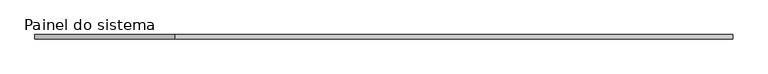
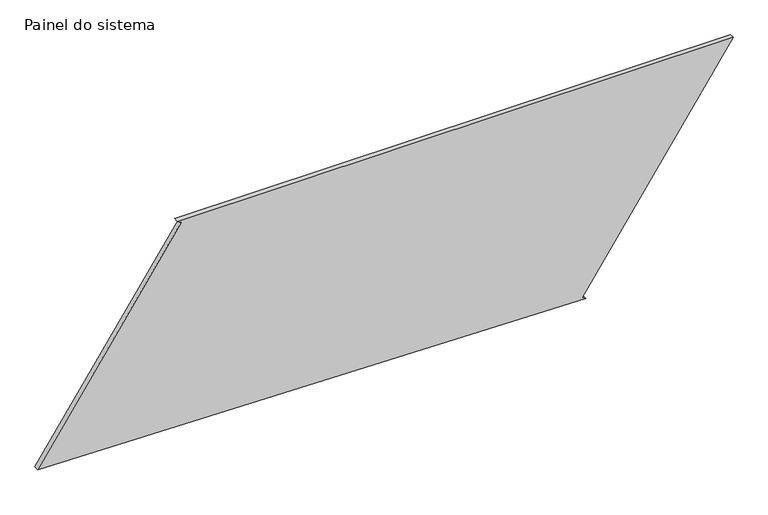
"""IFC4 building model written with IfcOpenShell, lengths in millimetres: plate geometry, Painel do sistema : Envidraçado."""

from ifc_helpers import new_model, si_unit, frame, origin, place, context, project, spatial, polyline, outline, extrude, source, transform, mapped, element, save


def painel_do_sistema_af02fa23(model_context):
    return source(origin(), model_context, "Body", "SweptSolid", [
        extrude(outline(polyline([(0.0, 1111.2336003), (14.052453, 1090.5568364), (1245.812938, 1927.6924915), (1245.812938, -1152.6117457), (1231.7604851, -1131.9349818), (60.8837577, -1927.6924915), (0.0, 1111.2336003)])), frame((0.0, 24.5, 0.0), z_axis=(0.0, 1.0, 0.0), x_axis=(0.0, 0.0, 1.0)), (0.0, 0.0, 1.0), 25.0),
    ])


if __name__ == "__main__":
    model = new_model("IFC4")
    model_context = context("Model", 3, world=origin())
    ifc_project = project(units=[si_unit("LENGTHUNIT", "METRE", prefix="MILLI")], contexts=[model_context])
    site = spatial("IfcSite", under=ifc_project)
    building = spatial("IfcBuilding", under=site)
    placement = place(None, origin())
    painel_do_sistema_shape = painel_do_sistema_af02fa23(model_context)
    element("IfcPlate", 1, ObjectType="Painel do sistema : Envidraçado", at=placement, inside=building, context=model_context, shape_type="MappedRepresentation", body=[
        mapped(painel_do_sistema_shape, transform((0.0, 0.0, 0.0), x_axis=(1.0, 0.0, 0.0), y_axis=(0.0, 1.0, 0.0), z_axis=(0.0, 0.0, 1.0))),
    ])
    save(model, "model.ifc")

# Revit data of these elements
# Type "Painel do sistema : Envidraçado"
#   Construction Type Id = "GSP4R"
#   Analytic Construction = "Vidraça única Pilkington 1/8 pol"
#   Visual Light Transmittance = 0.9
#   Solar Heat Gain Coefficient = 0.86
#   Heat Transfer Coefficient (U) = 6.7069 W/(m²·K)
# Element 1 (IfcPlate, "Painel do sistema : Envidraçado")
#   Materials on its faces: "Vidro"
# Materials
#   "Vidro": class "Vidro", colour RGB 0 128 192, transparency 0.9, Description = "Vidro de sílica", Cost = 0
